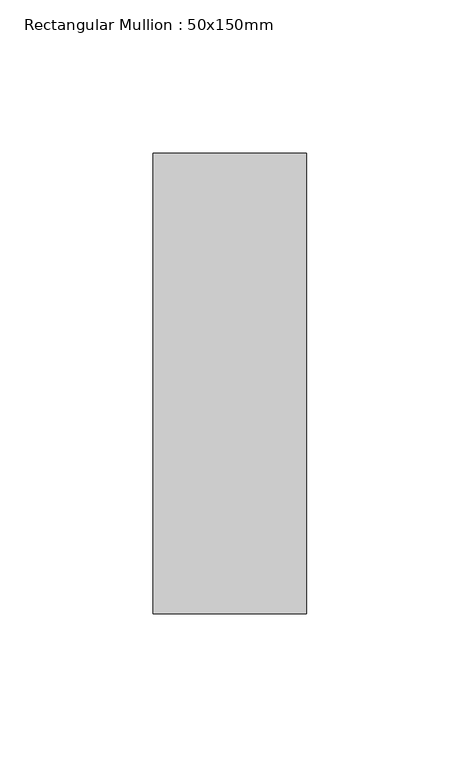
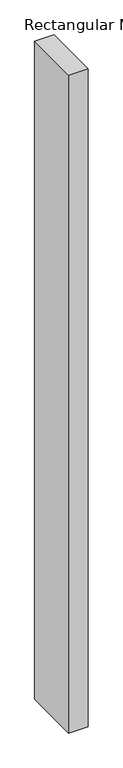
"""IFC4 building model written with IfcOpenShell, lengths in millimetres: member geometry, Rectangular Mullion : 50x150mm."""

import ifcopenshell
import ifcopenshell.guid

model = None  # the IFC model being written
_history = None  # IfcOwnerHistory: only IFC2X3 demands one
_inside = {}  # id of a spatial element -> (the spatial element, [elements in it])
_under = {}  # id of a project, library or spatial element -> (it, [spatial elements below it])
_declared = {}  # id of a project -> (the project, [libraries it declares])
_typed = {}  # id of a type object -> (the type object, [elements of that type])
_made_of = {}  # id of a material, layer set ... -> (it, [elements and type objects made of it])


def new_model(schema):
    """Start an empty IFC model of exactly this schema.

    Asked for "IFC4X3", IfcOpenShell would pick the latest addendum, in which some entities
    have other attributes; the version numbers below select the first issue.
    IFC2X3 requires an IfcOwnerHistory on every rooted entity: one is made here for all.
    """
    global model, _history
    if schema == "IFC4X3":
        model = ifcopenshell.file(schema_version=(4, 3, 0, 0))
    else:
        model = ifcopenshell.file(schema=schema)
    _inside.clear()
    _under.clear()
    _declared.clear()
    _typed.clear()
    _made_of.clear()
    _history = None
    if model.schema == "IFC2X3":
        org = make("IfcOrganization", Name="unknown")
        user = make(
            "IfcPersonAndOrganization",
            ThePerson=make("IfcPerson", FamilyName="unknown"),
            TheOrganization=org,
        )
        app = make(
            "IfcApplication",
            ApplicationDeveloper=org,
            Version="unknown",
            ApplicationFullName="unknown",
            ApplicationIdentifier="unknown",
        )
        _history = make(
            "IfcOwnerHistory",
            OwningUser=user,
            OwningApplication=app,
            ChangeAction="ADDED",
            CreationDate=0,
        )
    return model


def make(cls, **values):
    """One entity of the class cls with the attributes given. An attribute that is None is left unset."""
    return model.create_entity(
        cls, **{name: value for name, value in values.items() if value is not None}
    )


def rooted(cls, **values):
    """An entity with a GlobalId (a new one), such as an element, a storey or a relation."""
    return make(cls, GlobalId=ifcopenshell.guid.new(), OwnerHistory=_history, **values)


def si_unit(unit_type, name, prefix=None):
    """IfcSIUnit, for example si_unit("LENGTHUNIT", "METRE", prefix="MILLI")."""
    return make("IfcSIUnit", UnitType=unit_type, Prefix=prefix, Name=name)


def assignment(units):
    """IfcUnitAssignment: the units of a project."""
    return None if units is None else make("IfcUnitAssignment", Units=units)


def point(xyz):
    """IfcCartesianPoint."""
    return None if xyz is None else make("IfcCartesianPoint", Coordinates=xyz)


def direction(xyz):
    """IfcDirection."""
    return None if xyz is None else make("IfcDirection", DirectionRatios=xyz)


def frame(location, z_axis=None, x_axis=None):
    """IfcAxis2Placement3D, a coordinate frame: its origin and axes. An axis left out is left unset."""
    return make(
        "IfcAxis2Placement3D",
        Location=point(location),
        Axis=direction(z_axis),
        RefDirection=direction(x_axis),
    )


def origin():
    """The frame at (0, 0, 0) with its axes left unset."""
    return frame((0.0, 0.0, 0.0))


def place(relative_to, where):
    """IfcLocalPlacement: puts the frame where relative to a parent placement (None: the world)."""
    return make(
        "IfcLocalPlacement", PlacementRelTo=relative_to, RelativePlacement=where
    )


def context(
    kind, dimensions, precision=None, world=None, true_north=None, identifier=None
):
    """IfcGeometricRepresentationContext, for example the 3D "Model" context."""
    return make(
        "IfcGeometricRepresentationContext",
        ContextIdentifier=identifier,
        ContextType=kind,
        CoordinateSpaceDimension=dimensions,
        Precision=precision,
        WorldCoordinateSystem=world,
        TrueNorth=true_north,
    )


def project(units=None, contexts=None):
    """IfcProject with its units and contexts."""
    return rooted(
        "IfcProject",
        Name="project",
        RepresentationContexts=contexts,
        UnitsInContext=assignment(units),
    )


def spatial(cls, under=None, at=None, **own):
    """A site, building, storey or space (cls), placed at a placement, below another one or the project."""
    s = rooted(cls, ObjectPlacement=at, **own)
    if under is not None:
        _under.setdefault(under.id(), (under, []))[1].append(s)
    return s


def polyline(points):
    """IfcPolyline through the points."""
    return make("IfcPolyline", Points=[point(p) for p in points])


def outline(outer, holes=None, kind="AREA"):
    """IfcArbitraryClosedProfileDef: a profile drawn as a closed curve; with holes, ...WithVoids."""
    if holes is None:
        return make("IfcArbitraryClosedProfileDef", ProfileType=kind, OuterCurve=outer)
    return make(
        "IfcArbitraryProfileDefWithVoids",
        ProfileType=kind,
        OuterCurve=outer,
        InnerCurves=holes,
    )


def extrude(swept, where, along, depth):
    """IfcExtrudedAreaSolid: the profile swept, set in the frame where, extruded along a direction by depth."""
    return make(
        "IfcExtrudedAreaSolid",
        SweptArea=swept,
        Position=where,
        ExtrudedDirection=direction(along),
        Depth=depth,
    )


def shape(context_of_items, identifier, shape_type, items):
    """IfcShapeRepresentation: the items that make up one representation, for example the "Body"."""
    return make(
        "IfcShapeRepresentation",
        ContextOfItems=context_of_items,
        RepresentationIdentifier=identifier,
        RepresentationType=shape_type,
        Items=items,
    )


def source(mapping_origin, context_of_items, identifier, shape_type, items):
    """IfcRepresentationMap: a shape defined once, which mapped items show again and again."""
    return make(
        "IfcRepresentationMap",
        MappingOrigin=mapping_origin,
        MappedRepresentation=shape(context_of_items, identifier, shape_type, items),
    )


def transform(
    local_origin,
    x_axis=None,
    y_axis=None,
    z_axis=None,
    scale=None,
    scale2=None,
    scale3=None,
    uniform=True,
):
    """IfcCartesianTransformationOperator3D, or its non-uniform kind. x_axis, y_axis, z_axis: its Axis1, 2, 3."""
    if uniform:
        return make(
            "IfcCartesianTransformationOperator3D",
            Axis1=direction(x_axis),
            Axis2=direction(y_axis),
            LocalOrigin=point(local_origin),
            Scale=scale,
            Axis3=direction(z_axis),
        )
    return make(
        "IfcCartesianTransformationOperator3DnonUniform",
        Axis1=direction(x_axis),
        Axis2=direction(y_axis),
        LocalOrigin=point(local_origin),
        Scale=scale,
        Axis3=direction(z_axis),
        Scale2=scale2,
        Scale3=scale3,
    )


def mapped(mapping_source, mapping_target):
    """IfcMappedItem: shows the shape of a source again, moved by a transform."""
    return make(
        "IfcMappedItem", MappingSource=mapping_source, MappingTarget=mapping_target
    )


def made_of(thing, what):
    """Note that an element or type object is made of a material, layer set ...; save() writes the relation."""
    if what is not None:
        _made_of.setdefault(what.id(), (what, []))[1].append(thing)
    return thing


def element(
    cls,
    number,
    at=None,
    inside=None,
    cuts=None,
    type_object=None,
    material=None,
    context=None,
    identifier="Body",
    shape_type=None,
    held_by="IfcProductDefinitionShape",
    body=None,
    shapes=None,
    **own,
):
    """One element of the class cls, such as IfcWall. Its Tag is "e" and its number.

    at: its placement. inside: the storey or other place that contains it. cuts: it is an
    opening in that element (IfcRelVoidsElement). A single representation is given by context,
    identifier, shape_type and body (its items); several are given by shapes. held_by: the class
    of the entity that holds the representations. save() writes the other relations.
    """
    e = rooted(cls, Tag="e%d" % number, ObjectPlacement=at, **own)
    if body is not None:
        shapes = [shape(context, identifier, shape_type, body)]
    if shapes is not None:
        e.Representation = make(held_by, Representations=shapes)
    if inside is not None:
        _inside.setdefault(inside.id(), (inside, []))[1].append(e)
    if cuts is not None:
        rooted(
            "IfcRelVoidsElement", RelatingBuildingElement=cuts, RelatedOpeningElement=e
        )
    if type_object is not None:
        _typed.setdefault(type_object.id(), (type_object, []))[1].append(e)
    return made_of(e, material)


def aggregate(whole, parts):
    """IfcRelAggregates: a whole, such as a stair, and the parts it consists of."""
    return rooted("IfcRelAggregates", RelatingObject=whole, RelatedObjects=parts)


def save(model, path):
    """Write the relations noted so far, then the file.

    IfcRelAggregates (storeys below a building ...), IfcRelContainedInSpatialStructure (elements
    in a storey), IfcRelDefinesByType, IfcRelAssociatesMaterial and IfcRelDeclares: one each for
    every whole, place, type object, material and project.
    """
    for whole, parts in _under.values():
        aggregate(whole, parts)
    for where, things in _inside.values():
        rooted(
            "IfcRelContainedInSpatialStructure",
            RelatedElements=things,
            RelatingStructure=where,
        )
    for kind, things in _typed.values():
        rooted("IfcRelDefinesByType", RelatedObjects=things, RelatingType=kind)
    for what, things in _made_of.values():
        rooted("IfcRelAssociatesMaterial", RelatedObjects=things, RelatingMaterial=what)
    for by, libraries in _declared.values():
        rooted("IfcRelDeclares", RelatingContext=by, RelatedDefinitions=libraries)
    model.write(path)


def rectangular_mullion_50x150mm_ded00a16(model_context):
    return source(origin(), model_context, "Body", "SweptSolid", [
        extrude(outline(polyline([(0.0, 75.0), (0.0, -75.0), (-50.0, -75.0), (-50.0, 75.0), (0.0, 75.0)])), frame((0.0, 0.0, -1780.0), z_axis=(0.0, 0.0, 1.0), x_axis=(1.0, 0.0, 0.0)), (0.0, 0.0, 1.0), 1780.0),
    ])


if __name__ == "__main__":
    model = new_model("IFC4")
    model_context = context("Model", 3, world=origin())
    ifc_project = project(units=[si_unit("LENGTHUNIT", "METRE", prefix="MILLI")], contexts=[model_context])
    site = spatial("IfcSite", under=ifc_project)
    building = spatial("IfcBuilding", under=site)
    placement = place(None, origin())
    rectangular_mullion_50x150mm_shape = rectangular_mullion_50x150mm_ded00a16(model_context)
    element("IfcMember", 1, ObjectType="Rectangular Mullion : 50x150mm", at=placement, inside=building, context=model_context, shape_type="MappedRepresentation", body=[
        mapped(rectangular_mullion_50x150mm_shape, transform((0.0, 0.0, 0.0), x_axis=(1.0, 0.0, 0.0), y_axis=(0.0, 1.0, 0.0), z_axis=(0.0, 0.0, 1.0))),
    ])
    save(model, "model.ifc")

# Revit data of these elements
# Type "Rectangular Mullion : 50x150mm"
#   Keynote = "H11"
#   built-in parameter 1007304 = 0.492126 (stored number, unit not read)
#   built-in parameter 1007301 = 0.082021 (stored number, unit not read)
#   built-in parameter 1007300 = 0.082021 (stored number, unit not read)
# Element 1 (IfcMember, "Rectangular Mullion : 50x150mm")
#   Materials on its faces: "Aluminium"
# Materials
#   "Aluminium": class "Metal", colour RGB 247 247 247, transparency 0, Description = "Aluminium 6061", Cost = 0
